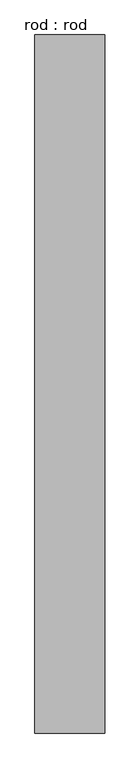
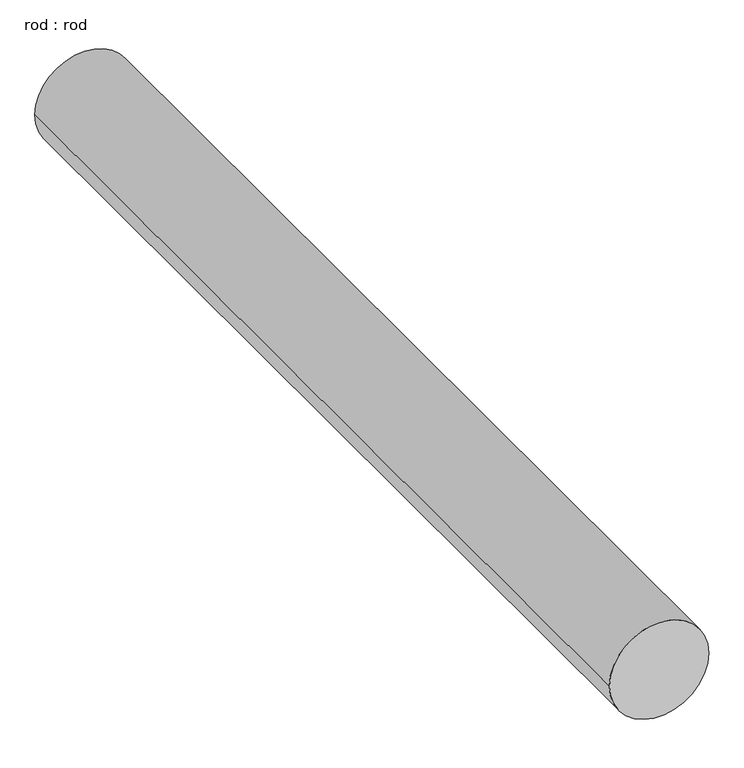
"""IFC4 building model written with IfcOpenShell, lengths in millimetres: proxy geometry, rod : rod."""

from ifc_helpers import new_model, si_unit, point, frame, frame_2d, origin, place, context, project, spatial, circle_curve, trimmed, segment, composite_curve, outline, extrude, source, transform, mapped, element, save


def rod_rod_b0117c38(model_context):
    return source(origin(), model_context, "Body", "SweptSolid", [
        extrude(outline(composite_curve([segment(trimmed(circle_curve(frame_2d((0.0108462, 0.0)), 200.0), [point((0.0108462, 200.0))], [point((0.0108462, -200.0))], False, "CARTESIAN"), True, "CONTINUOUS"), segment(trimmed(circle_curve(frame_2d((0.0108462, 0.0)), 200.0), [point((0.0108462, -200.0))], [point((0.0108462, 200.0))], False, "CARTESIAN"), True, "CONTINUOUS")], self_intersect=False)), frame((0.0, 2090.1911625, 0.0), z_axis=(0.0, 1.0, 0.0), x_axis=(0.0, 0.0, 1.0)), (0.0, 0.0, 1.0), 4005.0749057),
    ])


if __name__ == "__main__":
    model = new_model("IFC4")
    model_context = context("Model", 3, world=origin())
    ifc_project = project(units=[si_unit("LENGTHUNIT", "METRE", prefix="MILLI")], contexts=[model_context])
    site = spatial("IfcSite", under=ifc_project)
    building = spatial("IfcBuilding", under=site)
    placement = place(None, origin())
    rod_rod_shape = rod_rod_b0117c38(model_context)
    element("IfcBuildingElementProxy", 1, Name="rod : rod", ObjectType="rod : rod", at=placement, inside=building, context=model_context, shape_type="MappedRepresentation", body=[
        mapped(rod_rod_shape, transform((0.0, 0.0, 0.0), x_axis=(1.0, 0.0, 0.0), y_axis=(0.0, 1.0, 0.0), z_axis=(0.0, 0.0, 1.0))),
    ])
    save(model, "model.ifc")

# Revit data of these elements
# Type "rod : rod"
#   Default Elevation = 0
